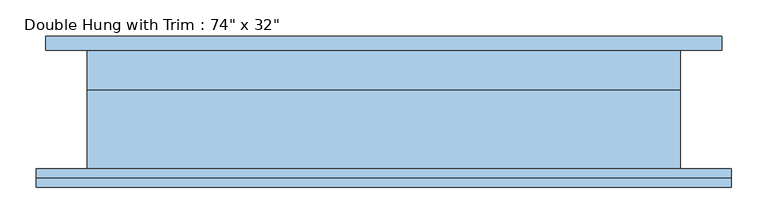
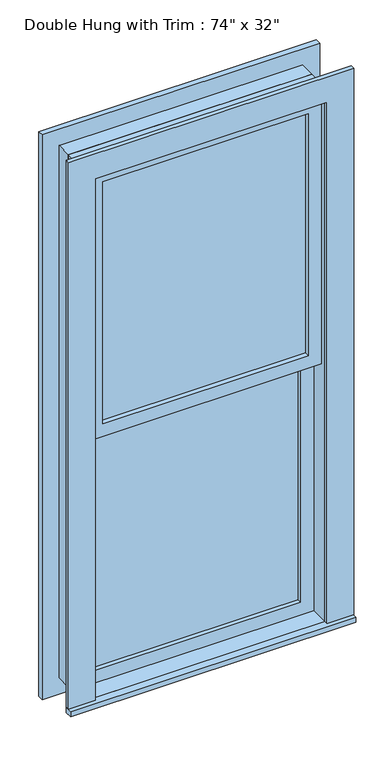
"""IFC4 building model written with IfcOpenShell, lengths in millimetres: window geometry."""

import ifcopenshell
import ifcopenshell.guid

model = None  # the IFC model being written
_history = None  # IfcOwnerHistory: only IFC2X3 demands one
_inside = {}  # id of a spatial element -> (the spatial element, [elements in it])
_under = {}  # id of a project, library or spatial element -> (it, [spatial elements below it])
_declared = {}  # id of a project -> (the project, [libraries it declares])
_typed = {}  # id of a type object -> (the type object, [elements of that type])
_made_of = {}  # id of a material, layer set ... -> (it, [elements and type objects made of it])


def new_model(schema):
    """Start an empty IFC model of exactly this schema.

    Asked for "IFC4X3", IfcOpenShell would pick the latest addendum, in which some entities
    have other attributes; the version numbers below select the first issue.
    IFC2X3 requires an IfcOwnerHistory on every rooted entity: one is made here for all.
    """
    global model, _history
    if schema == "IFC4X3":
        model = ifcopenshell.file(schema_version=(4, 3, 0, 0))
    else:
        model = ifcopenshell.file(schema=schema)
    _inside.clear()
    _under.clear()
    _declared.clear()
    _typed.clear()
    _made_of.clear()
    _history = None
    if model.schema == "IFC2X3":
        org = make("IfcOrganization", Name="unknown")
        user = make(
            "IfcPersonAndOrganization",
            ThePerson=make("IfcPerson", FamilyName="unknown"),
            TheOrganization=org,
        )
        app = make(
            "IfcApplication",
            ApplicationDeveloper=org,
            Version="unknown",
            ApplicationFullName="unknown",
            ApplicationIdentifier="unknown",
        )
        _history = make(
            "IfcOwnerHistory",
            OwningUser=user,
            OwningApplication=app,
            ChangeAction="ADDED",
            CreationDate=0,
        )
    return model


def make(cls, **values):
    """One entity of the class cls with the attributes given. An attribute that is None is left unset."""
    return model.create_entity(
        cls, **{name: value for name, value in values.items() if value is not None}
    )


def rooted(cls, **values):
    """An entity with a GlobalId (a new one), such as an element, a storey or a relation."""
    return make(cls, GlobalId=ifcopenshell.guid.new(), OwnerHistory=_history, **values)


def si_unit(unit_type, name, prefix=None):
    """IfcSIUnit, for example si_unit("LENGTHUNIT", "METRE", prefix="MILLI")."""
    return make("IfcSIUnit", UnitType=unit_type, Prefix=prefix, Name=name)


def assignment(units):
    """IfcUnitAssignment: the units of a project."""
    return None if units is None else make("IfcUnitAssignment", Units=units)


def point(xyz):
    """IfcCartesianPoint."""
    return None if xyz is None else make("IfcCartesianPoint", Coordinates=xyz)


def direction(xyz):
    """IfcDirection."""
    return None if xyz is None else make("IfcDirection", DirectionRatios=xyz)


def frame(location, z_axis=None, x_axis=None):
    """IfcAxis2Placement3D, a coordinate frame: its origin and axes. An axis left out is left unset."""
    return make(
        "IfcAxis2Placement3D",
        Location=point(location),
        Axis=direction(z_axis),
        RefDirection=direction(x_axis),
    )


def origin():
    """The frame at (0, 0, 0) with its axes left unset."""
    return frame((0.0, 0.0, 0.0))


def place(relative_to, where):
    """IfcLocalPlacement: puts the frame where relative to a parent placement (None: the world)."""
    return make(
        "IfcLocalPlacement", PlacementRelTo=relative_to, RelativePlacement=where
    )


def context(
    kind, dimensions, precision=None, world=None, true_north=None, identifier=None
):
    """IfcGeometricRepresentationContext, for example the 3D "Model" context."""
    return make(
        "IfcGeometricRepresentationContext",
        ContextIdentifier=identifier,
        ContextType=kind,
        CoordinateSpaceDimension=dimensions,
        Precision=precision,
        WorldCoordinateSystem=world,
        TrueNorth=true_north,
    )


def project(units=None, contexts=None):
    """IfcProject with its units and contexts."""
    return rooted(
        "IfcProject",
        Name="project",
        RepresentationContexts=contexts,
        UnitsInContext=assignment(units),
    )


def spatial(cls, under=None, at=None, **own):
    """A site, building, storey or space (cls), placed at a placement, below another one or the project."""
    s = rooted(cls, ObjectPlacement=at, **own)
    if under is not None:
        _under.setdefault(under.id(), (under, []))[1].append(s)
    return s


def polyline(points):
    """IfcPolyline through the points."""
    return make("IfcPolyline", Points=[point(p) for p in points])


def outline(outer, holes=None, kind="AREA"):
    """IfcArbitraryClosedProfileDef: a profile drawn as a closed curve; with holes, ...WithVoids."""
    if holes is None:
        return make("IfcArbitraryClosedProfileDef", ProfileType=kind, OuterCurve=outer)
    return make(
        "IfcArbitraryProfileDefWithVoids",
        ProfileType=kind,
        OuterCurve=outer,
        InnerCurves=holes,
    )


def extrude(swept, where, along, depth):
    """IfcExtrudedAreaSolid: the profile swept, set in the frame where, extruded along a direction by depth."""
    return make(
        "IfcExtrudedAreaSolid",
        SweptArea=swept,
        Position=where,
        ExtrudedDirection=direction(along),
        Depth=depth,
    )


def shape(context_of_items, identifier, shape_type, items):
    """IfcShapeRepresentation: the items that make up one representation, for example the "Body"."""
    return make(
        "IfcShapeRepresentation",
        ContextOfItems=context_of_items,
        RepresentationIdentifier=identifier,
        RepresentationType=shape_type,
        Items=items,
    )


def source(mapping_origin, context_of_items, identifier, shape_type, items):
    """IfcRepresentationMap: a shape defined once, which mapped items show again and again."""
    return make(
        "IfcRepresentationMap",
        MappingOrigin=mapping_origin,
        MappedRepresentation=shape(context_of_items, identifier, shape_type, items),
    )


def transform(
    local_origin,
    x_axis=None,
    y_axis=None,
    z_axis=None,
    scale=None,
    scale2=None,
    scale3=None,
    uniform=True,
):
    """IfcCartesianTransformationOperator3D, or its non-uniform kind. x_axis, y_axis, z_axis: its Axis1, 2, 3."""
    if uniform:
        return make(
            "IfcCartesianTransformationOperator3D",
            Axis1=direction(x_axis),
            Axis2=direction(y_axis),
            LocalOrigin=point(local_origin),
            Scale=scale,
            Axis3=direction(z_axis),
        )
    return make(
        "IfcCartesianTransformationOperator3DnonUniform",
        Axis1=direction(x_axis),
        Axis2=direction(y_axis),
        LocalOrigin=point(local_origin),
        Scale=scale,
        Axis3=direction(z_axis),
        Scale2=scale2,
        Scale3=scale3,
    )


def mapped(mapping_source, mapping_target):
    """IfcMappedItem: shows the shape of a source again, moved by a transform."""
    return make(
        "IfcMappedItem", MappingSource=mapping_source, MappingTarget=mapping_target
    )


def made_of(thing, what):
    """Note that an element or type object is made of a material, layer set ...; save() writes the relation."""
    if what is not None:
        _made_of.setdefault(what.id(), (what, []))[1].append(thing)
    return thing


def element(
    cls,
    number,
    at=None,
    inside=None,
    cuts=None,
    type_object=None,
    material=None,
    context=None,
    identifier="Body",
    shape_type=None,
    held_by="IfcProductDefinitionShape",
    body=None,
    shapes=None,
    **own,
):
    """One element of the class cls, such as IfcWall. Its Tag is "e" and its number.

    at: its placement. inside: the storey or other place that contains it. cuts: it is an
    opening in that element (IfcRelVoidsElement). A single representation is given by context,
    identifier, shape_type and body (its items); several are given by shapes. held_by: the class
    of the entity that holds the representations. save() writes the other relations.
    """
    e = rooted(cls, Tag="e%d" % number, ObjectPlacement=at, **own)
    if body is not None:
        shapes = [shape(context, identifier, shape_type, body)]
    if shapes is not None:
        e.Representation = make(held_by, Representations=shapes)
    if inside is not None:
        _inside.setdefault(inside.id(), (inside, []))[1].append(e)
    if cuts is not None:
        rooted(
            "IfcRelVoidsElement", RelatingBuildingElement=cuts, RelatedOpeningElement=e
        )
    if type_object is not None:
        _typed.setdefault(type_object.id(), (type_object, []))[1].append(e)
    return made_of(e, material)


def aggregate(whole, parts):
    """IfcRelAggregates: a whole, such as a stair, and the parts it consists of."""
    return rooted("IfcRelAggregates", RelatingObject=whole, RelatedObjects=parts)


def save(model, path):
    """Write the relations noted so far, then the file.

    IfcRelAggregates (storeys below a building ...), IfcRelContainedInSpatialStructure (elements
    in a storey), IfcRelDefinesByType, IfcRelAssociatesMaterial and IfcRelDeclares: one each for
    every whole, place, type object, material and project.
    """
    for whole, parts in _under.values():
        aggregate(whole, parts)
    for where, things in _inside.values():
        rooted(
            "IfcRelContainedInSpatialStructure",
            RelatedElements=things,
            RelatingStructure=where,
        )
    for kind, things in _typed.values():
        rooted("IfcRelDefinesByType", RelatedObjects=things, RelatingType=kind)
    for what, things in _made_of.values():
        rooted("IfcRelAssociatesMaterial", RelatedObjects=things, RelatingMaterial=what)
    for by, libraries in _declared.values():
        rooted("IfcRelDeclares", RelatingContext=by, RelatedDefinitions=libraries)
    model.write(path)


def window_7f3808cf(model_context):
    return source(origin(), model_context, "Body", "SweptSolid", [
        extrude(outline(polyline([(-342.9, -1.5875), (-342.9, 11.1125), (342.9, 11.1125), (342.9, -1.5875), (-342.9, -1.5875)])), frame((0.0, 0.0, 571.5), z_axis=(0.0, 0.0, 1.0), x_axis=(1.0, 0.0, 0.0)), (0.0, 0.0, 1.0), 854.075),
        extrude(outline(polyline([(1470.025, -387.35), (527.05, -387.35), (527.05, 387.35), (1470.025, 387.35), (1470.025, -387.35)]), holes=[polyline([(1425.575, -342.9), (1425.575, 342.9), (571.5, 342.9), (571.5, -342.9), (1425.575, -342.9)])]), frame((0.0, -17.4625, 0.0), z_axis=(0.0, 1.0, 0.0), x_axis=(0.0, 0.0, 1.0)), (0.0, 0.0, 1.0), 44.45),
        extrude(outline(polyline([(-476.25, -106.3625), (-476.25, -80.9625), (476.25, -80.9625), (476.25, -106.3625), (-476.25, -106.3625)])), frame((0.0, 0.0, 508.0), z_axis=(0.0, 0.0, 1.0), x_axis=(1.0, 0.0, 0.0)), (0.0, 0.0, 1.0), 19.05),
        extrude(outline(polyline([(2368.55, -387.35), (2368.55, 387.35), (527.05, 387.35), (527.05, 476.25), (2457.45, 476.25), (2457.45, -476.25), (527.05, -476.25), (527.05, -387.35), (2368.55, -387.35)])), frame((0.0, -93.6625, 0.0), z_axis=(0.0, 1.0, 0.0), x_axis=(0.0, 0.0, 1.0)), (0.0, 0.0, 1.0), 12.7),
        extrude(outline(polyline([(2444.75, 463.55), (2444.75, -463.55), (450.85, -463.55), (450.85, 463.55), (2444.75, 463.55)]), holes=[polyline([(2355.85, 374.65), (539.75, 374.65), (539.75, -374.65), (2355.85, -374.65), (2355.85, 374.65)])]), frame((0.0, 80.9625, 0.0), z_axis=(0.0, 1.0, 0.0), x_axis=(0.0, 0.0, 1.0)), (0.0, 0.0, 1.0), 19.05),
        extrude(outline(polyline([(342.9, -33.3375), (342.9, -46.0375), (-342.9, -46.0375), (-342.9, -33.3375), (342.9, -33.3375)])), frame((0.0, 0.0, 1470.025), z_axis=(0.0, 0.0, 1.0), x_axis=(1.0, 0.0, 0.0)), (0.0, 0.0, 1.0), 854.075),
        extrude(outline(polyline([(2368.55, -387.35), (1425.575, -387.35), (1425.575, 387.35), (2368.55, 387.35), (2368.55, -387.35)]), holes=[polyline([(2324.1, -342.9), (2324.1, 342.9), (1470.025, 342.9), (1470.025, -342.9), (2324.1, -342.9)])]), frame((0.0, -61.9125, 0.0), z_axis=(0.0, 1.0, 0.0), x_axis=(0.0, 0.0, 1.0)), (0.0, 0.0, 1.0), 44.45),
        extrude(outline(polyline([(2387.6, -406.4), (508.0, -406.4), (508.0, 406.4), (2387.6, 406.4), (2387.6, -406.4)]), holes=[polyline([(2355.85, -374.65), (2355.85, 374.65), (539.75, 374.65), (539.75, -374.65), (2355.85, -374.65)])]), frame((0.0, 26.9875, 0.0), z_axis=(0.0, 1.0, 0.0), x_axis=(0.0, 0.0, 1.0)), (0.0, 0.0, 1.0), 53.975),
        extrude(outline(polyline([(2387.6, 406.4), (2387.6, -406.4), (508.0, -406.4), (508.0, 406.4), (2387.6, 406.4)]), holes=[polyline([(2368.55, 387.35), (527.05, 387.35), (527.05, -387.35), (2368.55, -387.35), (2368.55, 387.35)])]), frame((0.0, -80.9625, 0.0), z_axis=(0.0, 1.0, 0.0), x_axis=(0.0, 0.0, 1.0)), (0.0, 0.0, 1.0), 107.95),
    ])


if __name__ == "__main__":
    model = new_model("IFC4")
    model_context = context("Model", 3, world=origin())
    ifc_project = project(units=[si_unit("LENGTHUNIT", "METRE", prefix="MILLI")], contexts=[model_context])
    site = spatial("IfcSite", under=ifc_project)
    building = spatial("IfcBuilding", under=site)
    placement = place(None, origin())
    window_shape = window_7f3808cf(model_context)
    element("IfcWindow", 1, ObjectType="Double Hung with Trim : 74\" x 32\"", at=placement, inside=building, context=model_context, shape_type="MappedRepresentation", body=[
        mapped(window_shape, transform((0.0, 0.0, 0.0), x_axis=(1.0, 0.0, 0.0), y_axis=(0.0, 1.0, 0.0), z_axis=(0.0, 0.0, 1.0))),
    ])
    save(model, "model.ifc")

# Revit data of these elements
# Type "Double Hung with Trim : 74\" x 32\""
#   Type Mark = "55"
#   COBie.Type.CreatedBy = "doug.wood@us.ibm.com"
#   COBie.Type.CreatedOn = "2016-04-14T02:07:26"
#   COBie.Type.Name = "Windows_Double Hung with Trim_74\" x 32\"_55"
#   COBie.Type.Category = "23-30 20 17 17 14 : Double-Hung Windows"
#   COBie.Type.Description = "Double Hung with Trim_74\" x 32\""
#   COBie.Type.Manufacturer = ""
#   COBie.Type.ModelNumber = ""
#   Construction Type Id = "GSP4R"
#   Assembly Code = "B2020100"
#   Analytic Construction = "1/8 in Pilkington single glazing"
#   COBie.Type.ReplacementCost = 0
#   Visual Light Transmittance = 0.9
#   Solar Heat Gain Coefficient = 0.78
#   Heat Transfer Coefficient (U) = 3.6886 W/(m²·K)
#   Height = 6' - 2"
#   Default Sill Height = 1' - 8"
#   Trim Projection - Ext. = 0' - 0 1/2"
#   Trim Projection - Int. = 0' - 0 3/4"
#   Trim Width - Exterior = 0' - 3 1/2"
#   Trim Width - Interior = 0' - 3 1/2"
#   Width = 2' - 8"
#   Window Inset = 0' - 0 3/4"
#   COBie.Type = no
#   Glass Pane Material = Glass
#   Sash Material = Sash - White
#   Trim Exterior Material = Trim - White
#   Trim Interior Material = Trim - White
#   Wall Closure = (empty or 0)
# Element 1 (IfcWindow, "Double Hung with Trim : 74\" x 32\"")
#   Materials on its faces: "Sash - White", "Trim - White", "Glass"
# Materials
#   "Glass": class "Glass", colour RGB 0 128 192, transparency 0.75, Description = "Soda Lime Glass", Cost = 0
#   "Sash - White": class "Wood", colour RGB 255 255 255, transparency 0, Cost = 0
#   "Trim - White": class "Wood", colour RGB 255 255 255, transparency 0, Cost = 0
